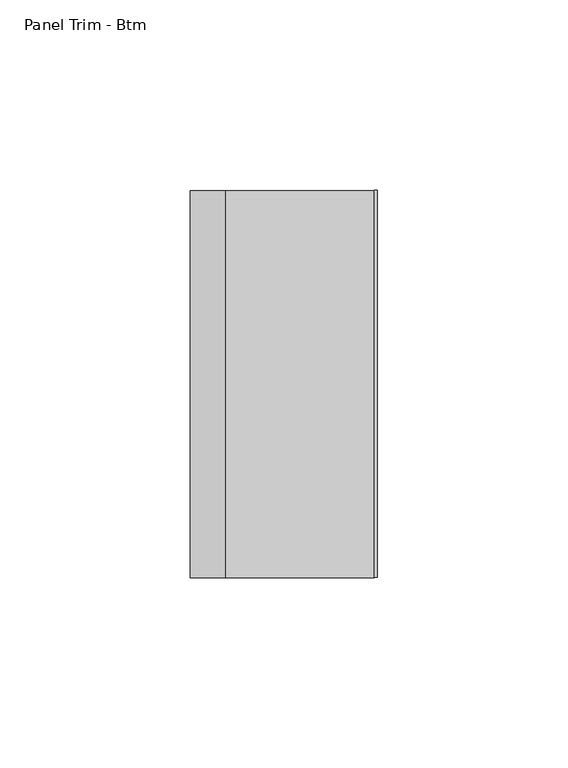
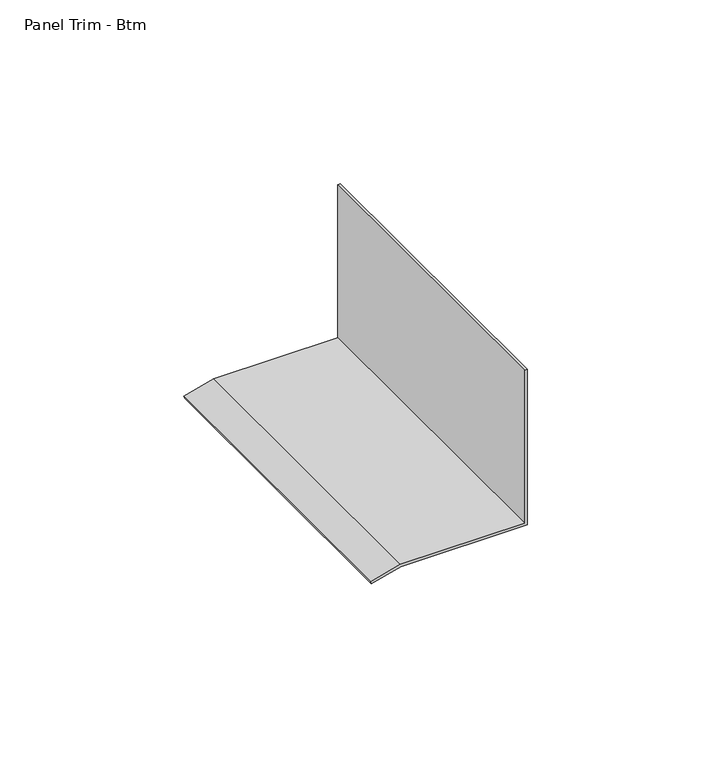
"""IFC4 building model written with IfcOpenShell, lengths in millimetres: proxy geometry, Btm Trim - Mull1 : Panel Trim - Btm."""

from ifc_helpers import new_model, si_unit, frame, origin, place, context, project, spatial, polyline, outline, extrude, source, transform, mapped, element, save


def panel_trim_btm_b3728a70(model_context):
    return source(origin(), model_context, "Body", "SweptSolid", [
        extrude(outline(polyline([(12.7, 587326.1141748), (10.2077022, 587316.8127928), (9.4409986, 587317.0182304), (11.90625, 587326.2186739), (11.90625, 587365.8934739), (63.5, 587365.8934739), (63.5, 587365.1060739), (12.7, 587365.1060739), (12.7, 587326.1141748)])), frame((0.0, -534096.6663841, 0.0), z_axis=(0.0, 1.0, 0.0), x_axis=(0.0, 0.0, 1.0)), (0.0, 0.0, 1.0), 101.6),
    ])


if __name__ == "__main__":
    model = new_model("IFC4")
    model_context = context("Model", 3, world=origin())
    ifc_project = project(units=[si_unit("LENGTHUNIT", "METRE", prefix="MILLI")], contexts=[model_context])
    site = spatial("IfcSite", under=ifc_project)
    building = spatial("IfcBuilding", under=site)
    placement = place(None, origin())
    panel_trim_btm_shape = panel_trim_btm_b3728a70(model_context)
    element("IfcBuildingElementProxy", 1, Name="Btm Trim - Mull1 : Panel Trim - Btm", ObjectType="Btm Trim - Mull1 : Panel Trim - Btm", at=placement, inside=building, context=model_context, shape_type="MappedRepresentation", body=[
        mapped(panel_trim_btm_shape, transform((0.0, 0.0, 0.0), x_axis=(1.0, 0.0, 0.0), y_axis=(0.0, 1.0, 0.0), z_axis=(0.0, 0.0, 1.0))),
    ])
    save(model, "model.ifc")

# Revit data of these elements
# Element 1 (IfcBuildingElementProxy, "Btm Trim - Mull1 : Panel Trim - Btm")
#   Materials on its faces: "BASE TRIM BY MTL PANEL MFR."
# Materials
#   "BASE TRIM BY MTL PANEL MFR.": class "Generic", colour RGB 239 242 240, transparency 0, Cost = 0
